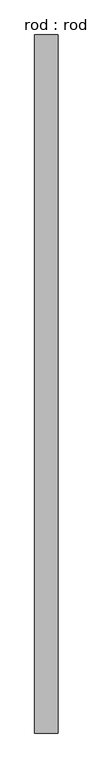
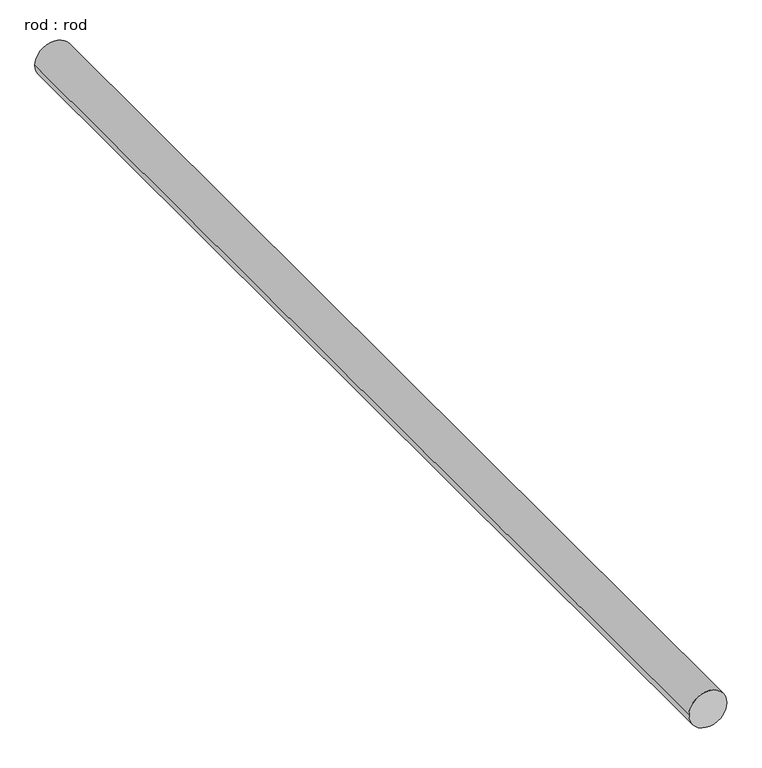
"""IFC4 building model written with IfcOpenShell, lengths in millimetres: proxy geometry, rod : rod."""

from ifc_helpers import new_model, si_unit, point, frame, frame_2d, origin, place, context, project, spatial, circle_curve, trimmed, segment, composite_curve, outline, extrude, source, transform, mapped, element, save


def rod_rod_01a77c82(model_context):
    return source(origin(), model_context, "Body", "SweptSolid", [
        extrude(outline(composite_curve([segment(trimmed(circle_curve(frame_2d((0.0108462, 0.0)), 200.0), [point((0.0108462, 200.0))], [point((0.0108462, -200.0))], False, "CARTESIAN"), True, "CONTINUOUS"), segment(trimmed(circle_curve(frame_2d((0.0108462, 0.0)), 200.0), [point((0.0108462, -200.0))], [point((0.0108462, 200.0))], False, "CARTESIAN"), True, "CONTINUOUS")], self_intersect=False)), frame((0.0, -1891.1502799, 0.0), z_axis=(0.0, 1.0, 0.0), x_axis=(0.0, 0.0, 1.0)), (0.0, 0.0, 1.0), 11967.7577904),
    ])


if __name__ == "__main__":
    model = new_model("IFC4")
    model_context = context("Model", 3, world=origin())
    ifc_project = project(units=[si_unit("LENGTHUNIT", "METRE", prefix="MILLI")], contexts=[model_context])
    site = spatial("IfcSite", under=ifc_project)
    building = spatial("IfcBuilding", under=site)
    placement = place(None, origin())
    rod_rod_shape = rod_rod_01a77c82(model_context)
    element("IfcBuildingElementProxy", 1, Name="rod : rod", ObjectType="rod : rod", at=placement, inside=building, context=model_context, shape_type="MappedRepresentation", body=[
        mapped(rod_rod_shape, transform((0.0, 0.0, 0.0), x_axis=(1.0, 0.0, 0.0), y_axis=(0.0, 1.0, 0.0), z_axis=(0.0, 0.0, 1.0))),
    ])
    save(model, "model.ifc")

# Revit data of these elements
# Project information
#   Project Issue Date = "Issue Date"
#   Project Status = "Project Status"
#   Client Name = "Owner"
#   Project Address = "Enter address here"
#   Project Name = "Project Name"
#   Project Number = "Project Number"
# Type "rod : rod"
#   Default Elevation = 0
